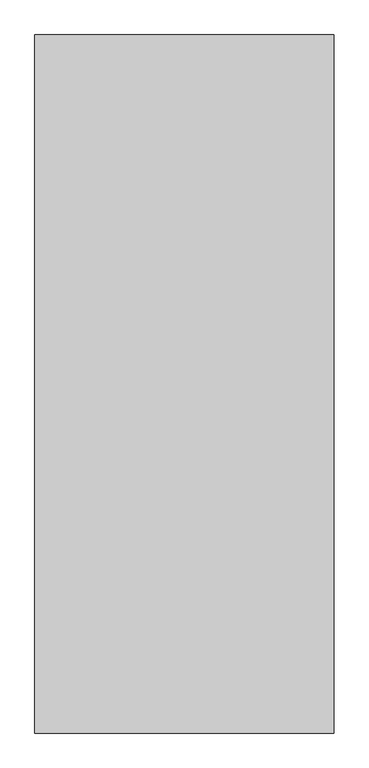
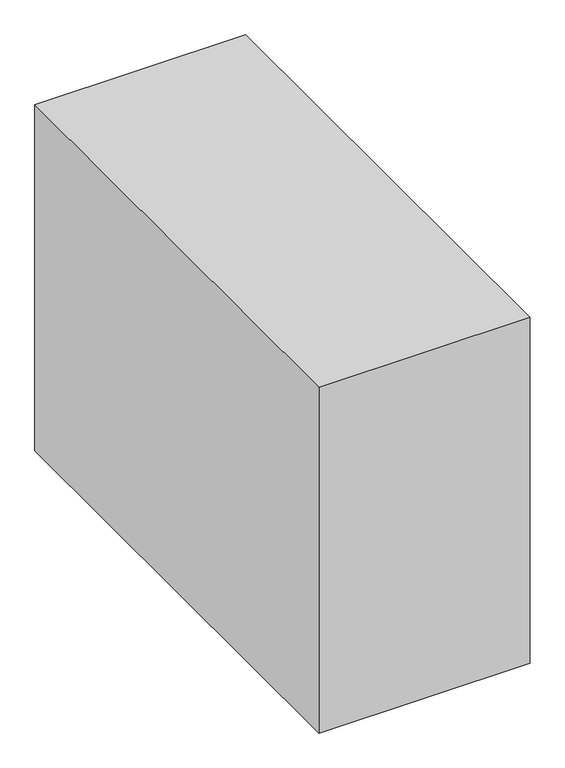
"""IFC4 building model written with IfcOpenShell, lengths in millimetres: proxy geometry, Space Planning Box_hec : Space Planning Box_hec."""

from ifc_helpers import new_model, si_unit, origin, origin_with_axes, place, context, project, spatial, polyline, outline, extrude, source, transform, mapped, element, save


def generic_models_2e4aee51(model_context):
    return source(origin(), model_context, "Body", "SweptSolid", [
        extrude(outline(polyline([(1500.0, 3500.0), (1500.0, -3500.0), (-1500.0, -3500.0), (-1500.0, 3500.0), (1500.0, 3500.0)])), origin_with_axes(), (0.0, 0.0, 1.0), 5200.0),
    ])


if __name__ == "__main__":
    model = new_model("IFC4")
    model_context = context("Model", 3, world=origin())
    ifc_project = project(units=[si_unit("LENGTHUNIT", "METRE", prefix="MILLI")], contexts=[model_context])
    site = spatial("IfcSite", under=ifc_project)
    building = spatial("IfcBuilding", under=site)
    placement = place(None, origin())
    generic_models_shape = generic_models_2e4aee51(model_context)
    element("IfcBuildingElementProxy", 1, Name="Space Planning Box_hec : Space Planning Box_hec", ObjectType="Space Planning Box_hec : Space Planning Box_hec", at=placement, inside=building, context=model_context, shape_type="MappedRepresentation", body=[
        mapped(generic_models_shape, transform((0.0, 0.0, 0.0), x_axis=(1.0, 0.0, 0.0), y_axis=(0.0, 1.0, 0.0), z_axis=(0.0, 0.0, 1.0))),
    ])
    save(model, "model.ifc")

# Revit data of these elements
# Type "Space Planning Box_hec : Space Planning Box_hec"
#   Type Comments = "..."
#   Room Name [instance default] = "?"
#   Interior Finish [instance default] = ""
#   Exterior Finish [instance default] = ""
#   Department [instance default] = ""
#   Assembly Code = "..."
#   ceiling height [instance default] = 0
#   Width [instance default] = 1524 mm
#   Program Area [instance default] = 0.00 m²
#   Length [instance default] = 1524 mm
#   Height [instance default] = 1524 mm
#   Area [instance default] = 2.32258 m²
#   Fill Color [instance default] = Cyan
#   Default Elevation = 0
# Element 1 (IfcBuildingElementProxy, "Space Planning Box_hec : Space Planning Box_hec")
#   Exterior Finish = "N/A..N/A,,EW1..N/A"
#   Department = "AR"
#   Width = 3000 mm
#   Program Area = 21.00 m²
#   Length = 7000 mm
#   Height = 5200 mm
#   Area = 21.00 m²
#   Materials on its faces: "Cyan"
# Materials
#   "Cyan": class "Generic", colour RGB 0 255 255, transparency 0.2, Cost = 0
